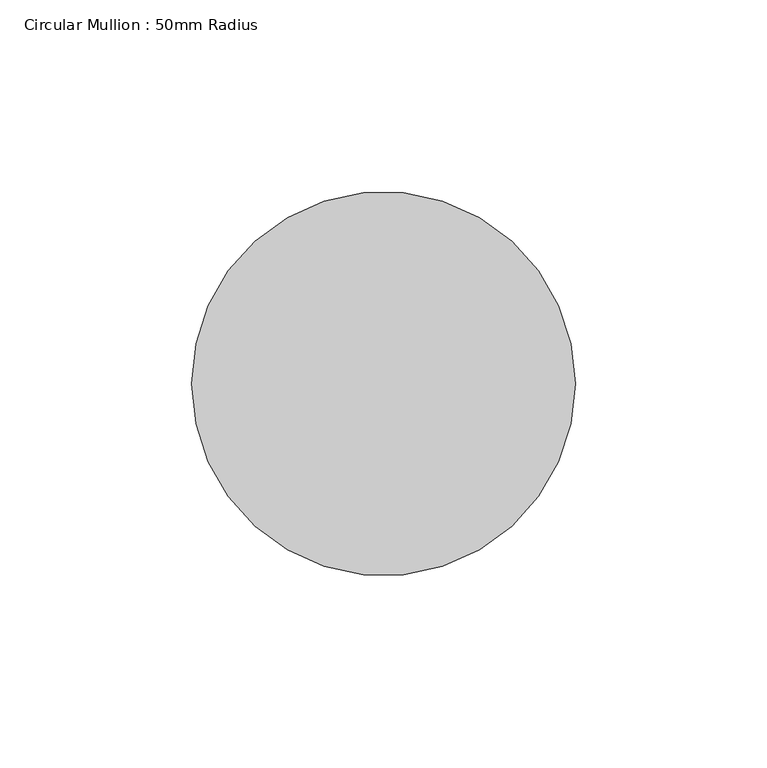
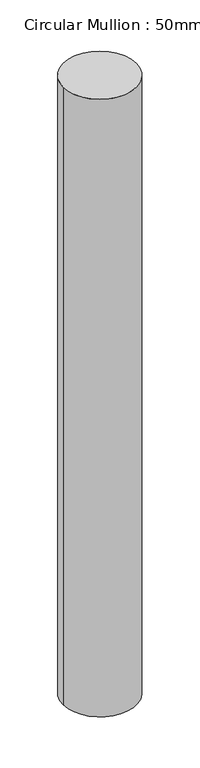
"""IFC4 building model written with IfcOpenShell, lengths in millimetres: member geometry, Circular Mullion : 50mm Radius."""

from ifc_helpers import new_model, si_unit, point, frame, origin, origin_2d, place, context, project, spatial, circle_curve, trimmed, segment, composite_curve, outline, extrude, source, transform, mapped, element, save


def circular_mullion_50mm_radius_8a24cf8c(model_context):
    return source(origin(), model_context, "Body", "SweptSolid", [
        extrude(outline(composite_curve([segment(trimmed(circle_curve(origin_2d(), 50.0), [point((50.0, 0.0))], [point((-50.0, 0.0))], False, "CARTESIAN"), True, "CONTINUOUS"), segment(trimmed(circle_curve(origin_2d(), 50.0), [point((-50.0, 0.0))], [point((50.0, 0.0))], False, "CARTESIAN"), True, "CONTINUOUS")], self_intersect=False)), frame((0.0, 0.0, -893.9186217), z_axis=(0.0, 0.0, 1.0), x_axis=(1.0, 0.0, 0.0)), (0.0, 0.0, 1.0), 893.9186217),
    ])


if __name__ == "__main__":
    model = new_model("IFC4")
    model_context = context("Model", 3, world=origin())
    ifc_project = project(units=[si_unit("LENGTHUNIT", "METRE", prefix="MILLI")], contexts=[model_context])
    site = spatial("IfcSite", under=ifc_project)
    building = spatial("IfcBuilding", under=site)
    placement = place(None, origin())
    circular_mullion_50mm_radius_shape = circular_mullion_50mm_radius_8a24cf8c(model_context)
    element("IfcMember", 1, ObjectType="Circular Mullion : 50mm Radius", at=placement, inside=building, context=model_context, shape_type="MappedRepresentation", body=[
        mapped(circular_mullion_50mm_radius_shape, transform((0.0, 0.0, 0.0), x_axis=(1.0, 0.0, 0.0), y_axis=(0.0, 1.0, 0.0), z_axis=(0.0, 0.0, 1.0))),
    ])
    save(model, "model.ifc")

# Revit data of these elements
# Type "Circular Mullion : 50mm Radius"
#   built-in parameter 1007350 = 0.164042 (stored number, unit not read)
# Element 1 (IfcMember, "Circular Mullion : 50mm Radius")
#   Materials on its faces: "Aluminium"
# Materials
#   "Aluminium": class "Metal", colour RGB 247 247 247, transparency 0, Description = "Aluminium 6061", Cost = 0
